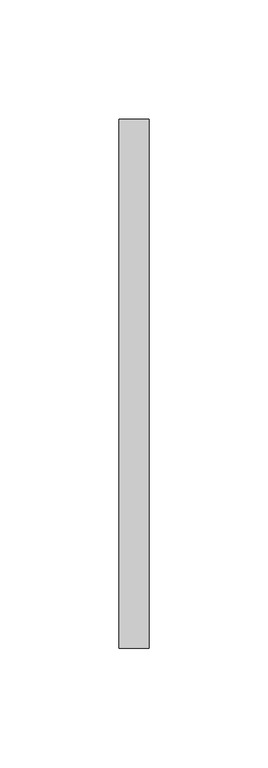
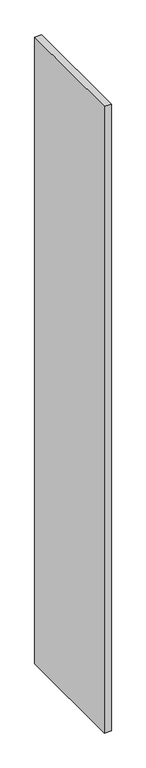
"""IFC4 building model written with IfcOpenShell, lengths in millimetres: proxy geometry, Inner panel:Inner panel:1:Inner panel:1 : Inner panel:Inner panel:300324:300043:Inner panel:1:Inner panel:1 : Inner panel:Inner panel:300324:300043 : Inner panel:Inner panel:1:Inner panel:1 : Inner panel:Inner panel:300324:300043:39 : Inner panel:Inner panel:1:Inner panel:1 : Inner panel:Inner panel:300324:300043:Inner panel:1:Inner panel:1 : Inner panel:Inner panel:300324:300043 : Inner panel:Inner panel:1:Inner panel:1 : Inner panel:Inner panel:300324:300043:300031."""

from ifc_helpers import new_model, si_unit, frame, origin, place, context, project, spatial, polyline, outline, extrude, source, transform, mapped, element, save


def generic_models_e5aa4141(model_context):
    return source(origin(), model_context, "Body", "SweptSolid", [
        extrude(outline(polyline([(560314.8617239, -579000.6913841), (560302.1617239, -579000.6913841), (560302.1617239, -578778.4413841), (560314.8617239, -578778.4413841), (560314.8617239, -579000.6913841)])), frame((0.0, 0.0, 4927.6), z_axis=(0.0, 0.0, 1.0), x_axis=(1.0, 0.0, 0.0)), (0.0, 0.0, 1.0), 1219.2),
    ])


if __name__ == "__main__":
    model = new_model("IFC4")
    model_context = context("Model", 3, world=origin())
    ifc_project = project(units=[si_unit("LENGTHUNIT", "METRE", prefix="MILLI")], contexts=[model_context])
    site = spatial("IfcSite", under=ifc_project)
    building = spatial("IfcBuilding", under=site)
    placement = place(None, origin())
    generic_models_shape = generic_models_e5aa4141(model_context)
    element("IfcBuildingElementProxy", 1, Name="Inner panel:Inner panel:1:Inner panel:1 : Inner panel:Inner panel:300324:300043:Inner panel:1:Inner panel:1 : Inner panel:Inner panel:300324:300043 : Inner panel:Inner panel:1:Inner panel:1 : Inner panel:Inner panel:300324:300043:39 : Inner panel:Inner panel:1:Inner panel:1 : Inner panel:Inner panel:300324:300043:Inner panel:1:Inner panel:1 : Inner panel:Inner panel:300324:300043 : Inner panel:Inner panel:1:Inner panel:1 : Inner panel:Inner panel:300324:300043:300031", ObjectType="Inner panel:Inner panel:1:Inner panel:1 : Inner panel:Inner panel:300324:300043:Inner panel:1:Inner panel:1 : Inner panel:Inner panel:300324:300043 : Inner panel:Inner panel:1:Inner panel:1 : Inner panel:Inner panel:300324:300043:39 : Inner panel:Inner panel:1:Inner panel:1 : Inner panel:Inner panel:300324:300043:Inner panel:1:Inner panel:1 : Inner panel:Inner panel:300324:300043 : Inner panel:Inner panel:1:Inner panel:1 : Inner panel:Inner panel:300324:300043:300031", at=placement, inside=building, context=model_context, shape_type="MappedRepresentation", body=[
        mapped(generic_models_shape, transform((0.0, 0.0, 0.0), x_axis=(1.0, 0.0, 0.0), y_axis=(0.0, 1.0, 0.0), z_axis=(0.0, 0.0, 1.0))),
    ])
    save(model, "model.ifc")

# Revit data of these elements
# Type "Inner panel:Inner panel:1:Inner panel:1 : Inner panel:Inner panel:300324:300043:Inner panel:1:Inner panel:1 : Inner panel:Inner panel:300324:300043 : Inner panel:Inner panel:1:Inner panel:1 : Inner panel:Inner panel:300324:300043:39 : Inner panel:Inner panel:1:Inner panel:1 : Inner panel:Inner panel:300324:300043:Inner panel:1:Inner panel:1 : Inner panel:Inner panel:300324:300043 : Inner panel:Inner panel:1:Inner panel:1 : Inner panel:Inner panel:300324:300043:300031"
#   NameOverride = "Inner panel:Inner panel:1:Inner panel:1 : Inner panel:Inner panel:300324:300043:Inner panel:1:Inner panel:1 : Inner panel:Inner panel:300324:300043 : Inner panel:Inner panel:1:Inner panel:1 : Inner panel:Inner panel:300324:300043:300031"
#   ObjectTypeOverride = "Inner panel:1:Inner panel:1 : Inner panel:Inner panel:300324:300043 : Inner panel:Inner panel:1:Inner panel:1 : Inner panel:Inner panel:300324:300043"
#   Reference = "Inner panel"
#   Tag = "300031"
# Element 1 (IfcBuildingElementProxy, "Inner panel:Inner panel:1:Inner panel:1 : Inner panel:Inner panel:300324:300043:Inner panel:1:Inner panel:1 : Inner panel:Inner panel:300324:300043 : Inner panel:Inner panel:1:Inner panel:1 : Inner panel:Inner panel:300324:300043:39 : Inner panel:Inner panel:1:Inner panel:1 : Inner panel:Inner panel:300324:300043:Inner panel:1:Inner panel:1 : Inner panel:Inner panel:300324:300043 : Inner panel:Inner panel:1:Inner panel:1 : Inner panel:Inner panel:300324:300043:300031")
#   Materials on its faces: "1/2\" EXTERIOR GRADE FIRE RETARDANT CDX PLYWOOD"
# Materials
#   "1/2\" EXTERIOR GRADE FIRE RETARDANT CDX PLYWOOD": class "Unassigned", colour RGB 196 177 123, transparency 0, Cost = 0
